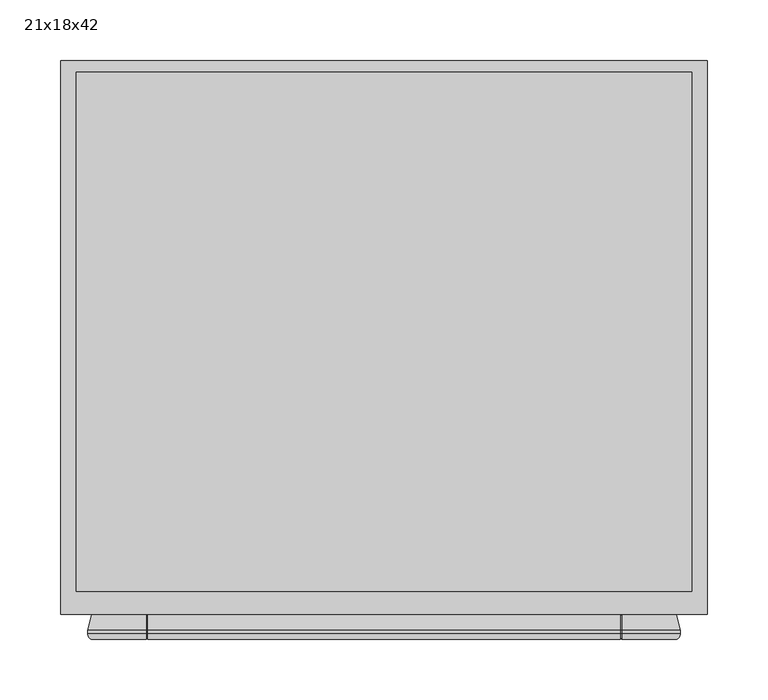
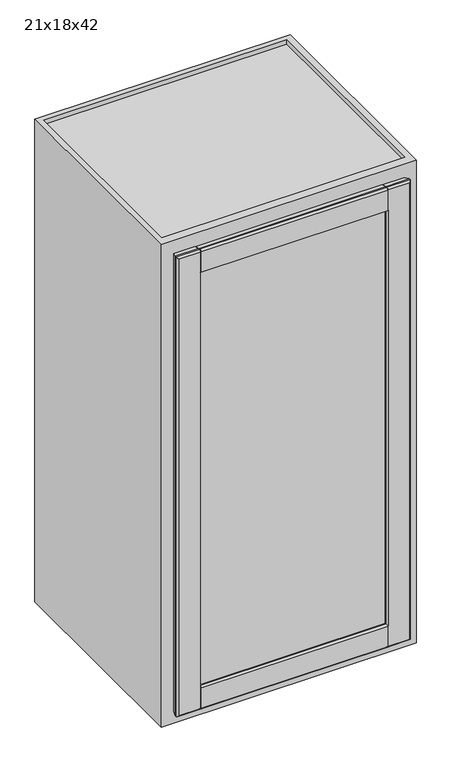
"""IFC4 building model written with IfcOpenShell, lengths in millimetres: furniture geometry, Cabinet-Wall-Merillat-Single_Door-Marlin : 21x18x42."""

import ifcopenshell
import ifcopenshell.guid

model = None  # the IFC model being written
_history = None  # IfcOwnerHistory: only IFC2X3 demands one
_inside = {}  # id of a spatial element -> (the spatial element, [elements in it])
_under = {}  # id of a project, library or spatial element -> (it, [spatial elements below it])
_declared = {}  # id of a project -> (the project, [libraries it declares])
_typed = {}  # id of a type object -> (the type object, [elements of that type])
_made_of = {}  # id of a material, layer set ... -> (it, [elements and type objects made of it])


def new_model(schema):
    """Start an empty IFC model of exactly this schema.

    Asked for "IFC4X3", IfcOpenShell would pick the latest addendum, in which some entities
    have other attributes; the version numbers below select the first issue.
    IFC2X3 requires an IfcOwnerHistory on every rooted entity: one is made here for all.
    """
    global model, _history
    if schema == "IFC4X3":
        model = ifcopenshell.file(schema_version=(4, 3, 0, 0))
    else:
        model = ifcopenshell.file(schema=schema)
    _inside.clear()
    _under.clear()
    _declared.clear()
    _typed.clear()
    _made_of.clear()
    _history = None
    if model.schema == "IFC2X3":
        org = make("IfcOrganization", Name="unknown")
        user = make(
            "IfcPersonAndOrganization",
            ThePerson=make("IfcPerson", FamilyName="unknown"),
            TheOrganization=org,
        )
        app = make(
            "IfcApplication",
            ApplicationDeveloper=org,
            Version="unknown",
            ApplicationFullName="unknown",
            ApplicationIdentifier="unknown",
        )
        _history = make(
            "IfcOwnerHistory",
            OwningUser=user,
            OwningApplication=app,
            ChangeAction="ADDED",
            CreationDate=0,
        )
    return model


def make(cls, **values):
    """One entity of the class cls with the attributes given. An attribute that is None is left unset."""
    return model.create_entity(
        cls, **{name: value for name, value in values.items() if value is not None}
    )


def rooted(cls, **values):
    """An entity with a GlobalId (a new one), such as an element, a storey or a relation."""
    return make(cls, GlobalId=ifcopenshell.guid.new(), OwnerHistory=_history, **values)


def si_unit(unit_type, name, prefix=None):
    """IfcSIUnit, for example si_unit("LENGTHUNIT", "METRE", prefix="MILLI")."""
    return make("IfcSIUnit", UnitType=unit_type, Prefix=prefix, Name=name)


def assignment(units):
    """IfcUnitAssignment: the units of a project."""
    return None if units is None else make("IfcUnitAssignment", Units=units)


def point(xyz):
    """IfcCartesianPoint."""
    return None if xyz is None else make("IfcCartesianPoint", Coordinates=xyz)


def direction(xyz):
    """IfcDirection."""
    return None if xyz is None else make("IfcDirection", DirectionRatios=xyz)


def frame(location, z_axis=None, x_axis=None):
    """IfcAxis2Placement3D, a coordinate frame: its origin and axes. An axis left out is left unset."""
    return make(
        "IfcAxis2Placement3D",
        Location=point(location),
        Axis=direction(z_axis),
        RefDirection=direction(x_axis),
    )


def origin():
    """The frame at (0, 0, 0) with its axes left unset."""
    return frame((0.0, 0.0, 0.0))


def place(relative_to, where):
    """IfcLocalPlacement: puts the frame where relative to a parent placement (None: the world)."""
    return make(
        "IfcLocalPlacement", PlacementRelTo=relative_to, RelativePlacement=where
    )


def context(
    kind, dimensions, precision=None, world=None, true_north=None, identifier=None
):
    """IfcGeometricRepresentationContext, for example the 3D "Model" context."""
    return make(
        "IfcGeometricRepresentationContext",
        ContextIdentifier=identifier,
        ContextType=kind,
        CoordinateSpaceDimension=dimensions,
        Precision=precision,
        WorldCoordinateSystem=world,
        TrueNorth=true_north,
    )


def project(units=None, contexts=None):
    """IfcProject with its units and contexts."""
    return rooted(
        "IfcProject",
        Name="project",
        RepresentationContexts=contexts,
        UnitsInContext=assignment(units),
    )


def spatial(cls, under=None, at=None, **own):
    """A site, building, storey or space (cls), placed at a placement, below another one or the project."""
    s = rooted(cls, ObjectPlacement=at, **own)
    if under is not None:
        _under.setdefault(under.id(), (under, []))[1].append(s)
    return s


def polyline(points):
    """IfcPolyline through the points."""
    return make("IfcPolyline", Points=[point(p) for p in points])


def circle_curve(where, radius):
    """IfcCircle in the frame where."""
    return make("IfcCircle", Position=where, Radius=radius)


def ellipse_curve(where, semi_axis1, semi_axis2):
    """IfcEllipse in the frame where."""
    return make(
        "IfcEllipse", Position=where, SemiAxis1=semi_axis1, SemiAxis2=semi_axis2
    )


def outline(outer, holes=None, kind="AREA"):
    """IfcArbitraryClosedProfileDef: a profile drawn as a closed curve; with holes, ...WithVoids."""
    if holes is None:
        return make("IfcArbitraryClosedProfileDef", ProfileType=kind, OuterCurve=outer)
    return make(
        "IfcArbitraryProfileDefWithVoids",
        ProfileType=kind,
        OuterCurve=outer,
        InnerCurves=holes,
    )


def extrude(swept, where, along, depth):
    """IfcExtrudedAreaSolid: the profile swept, set in the frame where, extruded along a direction by depth."""
    return make(
        "IfcExtrudedAreaSolid",
        SweptArea=swept,
        Position=where,
        ExtrudedDirection=direction(along),
        Depth=depth,
    )


def faces_of(points, faces, orient=None, outer=None):
    """IfcFace entities. A face is a list of loops; a loop is a list of indices into points, from 0.

    orient and outer hold one flag for each loop. By default every Orientation is true, the
    first loop of a face is its IfcFaceOuterBound and the others are IfcFaceBound.
    """
    made = []
    for i, loops in enumerate(faces):
        bounds = []
        for j, loop in enumerate(loops):
            is_outer = j == 0 if outer is None else outer[i][j]
            bounds.append(
                make(
                    "IfcFaceOuterBound" if is_outer else "IfcFaceBound",
                    Bound=make("IfcPolyLoop", Polygon=[points[k] for k in loop]),
                    Orientation=True if orient is None else orient[i][j],
                )
            )
        made.append(make("IfcFace", Bounds=bounds))
    return made


def faceted_brep(points, faces, orient=None, outer=None, voids=None):
    """IfcFacetedBrep: a solid bounded by flat faces; with voids (closed shells), ...WithVoids."""
    shared = [point(p) for p in points]
    hull = make("IfcClosedShell", CfsFaces=faces_of(shared, faces, orient, outer))
    if voids is None:
        return make("IfcFacetedBrep", Outer=hull)
    return make(
        "IfcFacetedBrepWithVoids",
        Outer=hull,
        Voids=[
            make(cls, CfsFaces=faces_of(shared, fs, o, b)) for cls, fs, o, b in voids
        ],
    )


def shape(context_of_items, identifier, shape_type, items):
    """IfcShapeRepresentation: the items that make up one representation, for example the "Body"."""
    return make(
        "IfcShapeRepresentation",
        ContextOfItems=context_of_items,
        RepresentationIdentifier=identifier,
        RepresentationType=shape_type,
        Items=items,
    )


def source(mapping_origin, context_of_items, identifier, shape_type, items):
    """IfcRepresentationMap: a shape defined once, which mapped items show again and again."""
    return make(
        "IfcRepresentationMap",
        MappingOrigin=mapping_origin,
        MappedRepresentation=shape(context_of_items, identifier, shape_type, items),
    )


def transform(
    local_origin,
    x_axis=None,
    y_axis=None,
    z_axis=None,
    scale=None,
    scale2=None,
    scale3=None,
    uniform=True,
):
    """IfcCartesianTransformationOperator3D, or its non-uniform kind. x_axis, y_axis, z_axis: its Axis1, 2, 3."""
    if uniform:
        return make(
            "IfcCartesianTransformationOperator3D",
            Axis1=direction(x_axis),
            Axis2=direction(y_axis),
            LocalOrigin=point(local_origin),
            Scale=scale,
            Axis3=direction(z_axis),
        )
    return make(
        "IfcCartesianTransformationOperator3DnonUniform",
        Axis1=direction(x_axis),
        Axis2=direction(y_axis),
        LocalOrigin=point(local_origin),
        Scale=scale,
        Axis3=direction(z_axis),
        Scale2=scale2,
        Scale3=scale3,
    )


def mapped(mapping_source, mapping_target):
    """IfcMappedItem: shows the shape of a source again, moved by a transform."""
    return make(
        "IfcMappedItem", MappingSource=mapping_source, MappingTarget=mapping_target
    )


def made_of(thing, what):
    """Note that an element or type object is made of a material, layer set ...; save() writes the relation."""
    if what is not None:
        _made_of.setdefault(what.id(), (what, []))[1].append(thing)
    return thing


def element(
    cls,
    number,
    at=None,
    inside=None,
    cuts=None,
    type_object=None,
    material=None,
    context=None,
    identifier="Body",
    shape_type=None,
    held_by="IfcProductDefinitionShape",
    body=None,
    shapes=None,
    **own,
):
    """One element of the class cls, such as IfcWall. Its Tag is "e" and its number.

    at: its placement. inside: the storey or other place that contains it. cuts: it is an
    opening in that element (IfcRelVoidsElement). A single representation is given by context,
    identifier, shape_type and body (its items); several are given by shapes. held_by: the class
    of the entity that holds the representations. save() writes the other relations.
    """
    e = rooted(cls, Tag="e%d" % number, ObjectPlacement=at, **own)
    if body is not None:
        shapes = [shape(context, identifier, shape_type, body)]
    if shapes is not None:
        e.Representation = make(held_by, Representations=shapes)
    if inside is not None:
        _inside.setdefault(inside.id(), (inside, []))[1].append(e)
    if cuts is not None:
        rooted(
            "IfcRelVoidsElement", RelatingBuildingElement=cuts, RelatedOpeningElement=e
        )
    if type_object is not None:
        _typed.setdefault(type_object.id(), (type_object, []))[1].append(e)
    return made_of(e, material)


def aggregate(whole, parts):
    """IfcRelAggregates: a whole, such as a stair, and the parts it consists of."""
    return rooted("IfcRelAggregates", RelatingObject=whole, RelatedObjects=parts)


def save(model, path):
    """Write the relations noted so far, then the file.

    IfcRelAggregates (storeys below a building ...), IfcRelContainedInSpatialStructure (elements
    in a storey), IfcRelDefinesByType, IfcRelAssociatesMaterial and IfcRelDeclares: one each for
    every whole, place, type object, material and project.
    """
    for whole, parts in _under.values():
        aggregate(whole, parts)
    for where, things in _inside.values():
        rooted(
            "IfcRelContainedInSpatialStructure",
            RelatedElements=things,
            RelatingStructure=where,
        )
    for kind, things in _typed.values():
        rooted("IfcRelDefinesByType", RelatedObjects=things, RelatingType=kind)
    for what, things in _made_of.values():
        rooted("IfcRelAssociatesMaterial", RelatedObjects=things, RelatingMaterial=what)
    for by, libraries in _declared.values():
        rooted("IfcRelDeclares", RelatingContext=by, RelatedDefinitions=libraries)
    model.write(path)


def plane_surface(at):
    """IfcPlane: the flat surface through the origin of the frame at, square to its z axis."""
    return make("IfcPlane", Position=at)


def cylinder_surface(at, radius):
    """IfcCylindricalSurface: all points at the distance radius from the z axis of the frame at."""
    return make("IfcCylindricalSurface", Position=at, Radius=radius)


def advanced_brep(points, edges, surfaces, faces):
    """IfcAdvancedBrep: a solid bounded by faces that lie on surfaces and meet in shared edges.

    An edge is (start, end): straight between two places in points (the first is 0);
    or (start, end, curve); or (start, end, curve, False) where it runs against its curve.
    A face is (place in surfaces, loops), or (place, loops, False) where it looks against
    its surface's normal. A loop lists edges by number (the first is 1), with a minus sign
    where the edge is run from its end to its start. The first loop is the outer one.
    """
    corners = [point(p) for p in points]
    vertices = [make("IfcVertexPoint", VertexGeometry=c) for c in corners]
    made = []
    for start, end, *more in edges:
        made.append(
            make(
                "IfcEdgeCurve",
                EdgeStart=vertices[start],
                EdgeEnd=vertices[end],
                EdgeGeometry=more[0] if more else make("IfcPolyline", Points=[corners[start], corners[end]]),
                SameSense=more[1] if len(more) > 1 else True,
            )
        )
    hull = []
    for where, loops, *sense in faces:
        bounds = []
        for j, loop in enumerate(loops):
            ring = [make("IfcOrientedEdge", EdgeElement=made[abs(k) - 1], Orientation=k > 0) for k in loop]
            bounds.append(
                make(
                    "IfcFaceOuterBound" if j == 0 else "IfcFaceBound",
                    Bound=make("IfcEdgeLoop", EdgeList=ring),
                    Orientation=True,
                )
            )
        hull.append(make("IfcAdvancedFace", Bounds=bounds, FaceSurface=surfaces[where], SameSense=sense[0] if sense else True))
    return make("IfcAdvancedBrep", Outer=make("IfcClosedShell", CfsFaces=hull))


def furniture_21x18x42_ea13cc69(model_context):
    return source(origin(), model_context, "Body", "SolidModel", [
        advanced_brep(
        [(-214.7038372, -534.9621, 2108.2), (-214.7038372, -534.9621, 1092.2), (-211.6073447, -539.4325, 1095.2964925), (-211.6073447, -539.4325, 2105.1035075), (-214.7038372, -532.1935, 2108.2), (-214.7038372, -532.1935, 1092.2), (-211.1986372, -519.1125, 2104.6948), (-211.1986372, -519.1125, 1095.7052), (-166.5026744, -519.1125, 2059.9988372), (-166.1325427, -519.90625, 2059.6287055), (-164.0513837, -524.36931, 2057.5475465), (-164.0513837, -524.36931, 1142.8524535), (-166.1325427, -519.90625, 1140.7712945), (-166.5026744, -519.1125, 1140.4011628), (-165.4511532, -526.6094093, 2058.947316), (-165.4511532, -526.6094093, 1141.452684), (-179.7788372, -526.8595, 2073.275), (-179.7788372, -526.8595, 1127.125), (-179.7788372, -531.6855, 2073.275), (-179.7788372, -531.6855, 1127.125), (-165.4511532, -531.9355907, 2058.947316), (-165.4511532, -531.9355907, 1141.452684), (-164.0513837, -534.17569, 2057.5475465), (-164.0513837, -534.17569, 1142.8524535), (-166.1325427, -538.63875, 2059.6287055), (-166.499807, -539.4263508, 2059.9959698), (-166.5026744, -539.4325, 1140.4011628), (-166.1325427, -538.63875, 1140.7712945), (271.1496703, -539.4325, 1095.2964925), (226.0819441, -539.4325, 1095.2964925), (226.0819441, -534.9621, 1092.2), (274.2461628, -534.9621, 1092.2), (-166.499807, -534.9621, 1092.2), (-166.499807, -539.4325, 1095.2964925), (-164.912307, -534.9621, 1092.2), (224.4944441, -534.9621, 1092.2), (224.4944441, -539.4325, 1095.2964925), (-164.912307, -539.4325, 1095.2964925), (226.0819441, -532.1935, 1092.2), (274.2461628, -532.1935, 1092.2), (-166.499807, -532.1935, 1092.2), (-164.912307, -532.1935, 1092.2), (224.4944441, -532.1935, 1092.2), (226.0819441, -519.1125, 1095.7052), (270.7409628, -519.1125, 1095.7052), (-166.499807, -519.1125, 1095.7052), (-164.912307, -519.1125, 1095.7052), (224.4944441, -519.1125, 1095.7052), (223.5937093, -524.36931, 1142.8524535), (225.6748683, -519.90625, 1140.7712945), (224.4944441, -519.90625, 1140.7712945), (224.4944441, -519.1125, 1140.4011628), (-164.912307, -519.1125, 1140.4011628), (-164.912307, -519.90625, 1140.7712945), (224.9934787, -526.6094093, 1141.452684), (239.3211628, -526.8595, 1127.125), (239.3211628, -531.6855, 1127.125), (224.9934787, -531.9355907, 1141.452684), (223.5937093, -534.17569, 1142.8524535), (-164.912307, -538.63875, 1140.7712945), (-164.912307, -539.4325, 1140.4011628), (224.4944441, -539.4325, 1140.4011628), (224.4944441, -538.63875, 1140.7712945), (225.6748683, -538.63875, 1140.7712945), (274.2461628, -534.9621, 2108.2), (271.1496703, -539.4325, 2105.1035075), (274.2461628, -532.1935, 2108.2), (270.7409628, -519.1125, 2104.6948), (226.045, -519.1125, 1140.4011628), (223.5937093, -524.36931, 2057.5475465), (225.6748683, -519.90625, 2059.6287055), (226.045, -519.1125, 2059.9988372), (224.9934787, -526.6094093, 2058.947316), (239.3211628, -526.8595, 2073.275), (239.3211628, -531.6855, 2073.275), (224.9934787, -531.9355907, 2058.947316), (223.5937093, -534.17569, 2057.5475465), (226.045, -539.4325, 1140.4011628), (226.045, -539.4325, 2059.9988372), (225.6748683, -538.63875, 2059.6287055), (-166.499807, -539.4325, 2105.1035075), (-166.499807, -534.9621, 2108.2), (226.0819441, -534.9621, 2108.2), (226.0819441, -539.4325, 2105.1035075), (224.4944441, -534.9621, 2108.2), (-164.912307, -534.9621, 2108.2), (-164.912307, -539.4325, 2105.1035075), (224.4944441, -539.4325, 2105.1035075), (-166.499807, -532.1935, 2108.2), (226.0819441, -532.1935, 2108.2), (224.4944441, -532.1935, 2108.2), (-164.912307, -532.1935, 2108.2), (-166.499807, -519.1125, 2104.6948), (226.0819441, -519.1125, 2104.6948), (224.4944441, -519.1125, 2104.6948), (-164.912307, -519.1125, 2104.6948), (224.4944441, -519.1125, 2059.9988372), (-164.912307, -519.1125, 2059.9988372), (-164.912307, -519.90625, 2059.6287055), (224.4944441, -519.90625, 2059.6287055), (224.4944441, -538.63875, 2059.6287055), (224.4944441, -539.4325, 2059.9988372), (-164.912307, -539.4325, 2059.9988372), (-164.912307, -538.63875, 2059.6287055), (224.4944441, -538.63875, 2104.9526052), (224.4944441, -534.9621, 2107.40625), (224.4944441, -532.2980037, 2107.40625), (224.4944441, -519.90625, 2104.0857412), (226.0819441, -519.90625, 2059.6287055), (226.0819441, -519.90625, 2104.0857412), (226.0819441, -532.2980037, 2107.40625), (226.0819441, -534.9621, 2107.40625), (226.0819441, -538.63875, 2104.9526052), (226.0819441, -538.63875, 2059.6287055), (-166.499807, -538.63875, 2059.6287055), (-166.499807, -538.63875, 2104.9526052), (-166.499807, -534.9621, 2107.40625), (-166.499807, -532.2980037, 2107.40625), (-166.499807, -519.90625, 2104.0857412), (-166.499807, -519.90625, 2059.6287055), (-164.912307, -519.90625, 2104.0857412), (-164.912307, -532.2980037, 2107.40625), (-164.912307, -534.9621, 2107.40625), (-164.912307, -538.63875, 2104.9526052), (-166.499807, -519.90625, 1140.7712945), (-166.499807, -519.90625, 1096.3142588), (-166.499807, -532.2980037, 1092.99375), (-166.499807, -534.9621, 1092.99375), (-166.499807, -538.63875, 1095.4473948), (-166.499807, -538.63875, 1140.7712945), (-164.912307, -538.63875, 1095.4473948), (-164.912307, -534.9621, 1092.99375), (-164.912307, -532.2980037, 1092.99375), (-164.912307, -519.90625, 1096.3142588), (224.4944441, -519.90625, 1096.3142588), (224.4944441, -532.2980037, 1092.99375), (224.4944441, -534.9621, 1092.99375), (224.4944441, -538.63875, 1095.4473948), (226.0819441, -538.63875, 1140.7712945), (226.0819441, -538.63875, 1095.4473948), (226.0819441, -534.9621, 1092.99375), (226.0819441, -532.2980037, 1092.99375), (226.0819441, -519.90625, 1096.3142588), (226.0819441, -519.90625, 1140.7712945)],
        [
            (0, 1),
            (1, 2, ellipse_curve(frame((-209.9286372, -534.9621, 1096.9752), z_axis=(-0.7071067811865475, 0.0, 0.7071067811865475), x_axis=(0.7071067811865474, 0.0, 0.7071067811865476)), 6.7531526, 4.7752)),
            (2, 3),
            (3, 0, ellipse_curve(frame((-209.9286372, -534.9621, 2103.4248), z_axis=(-0.7071067811865475, 0.0, -0.7071067811865475), x_axis=(-0.7071067811865474, 0.0, 0.7071067811865476)), 6.7531526, 4.7752)),
            (0, 4),
            (4, 5),
            (5, 1),
            (4, 6),
            (6, 7),
            (7, 5),
            (8, 9),
            (9, 10),
            (10, 11),
            (11, 12),
            (12, 13),
            (13, 8),
            (10, 14, ellipse_curve(frame((-165.4786372, -525.0348492, 2058.9748), z_axis=(-0.7071067811865475, 0.0, -0.7071067811865475), x_axis=(-0.7071067811865474, 0.0, 0.7071067811865476)), 2.2271035, 1.5748)),
            (14, 15),
            (15, 11, ellipse_curve(frame((-165.4786372, -525.0348492, 1141.4252), z_axis=(-0.7071067811865475, 0.0, 0.7071067811865475), x_axis=(0.7071067811865474, 0.0, 0.7071067811865476)), 2.2271035, 1.5748)),
            (14, 16),
            (16, 17),
            (17, 15),
            (16, 18),
            (18, 19),
            (19, 17),
            (18, 20),
            (20, 21),
            (21, 19),
            (20, 22, ellipse_curve(frame((-165.4786372, -533.5101508, 2058.9748), z_axis=(-0.7071067811865475, 0.0, -0.7071067811865475), x_axis=(-0.7071067811865474, 0.0, 0.7071067811865476)), 2.2271035, 1.5748)),
            (22, 23),
            (23, 21, ellipse_curve(frame((-165.4786372, -533.5101508, 1141.4252), z_axis=(-0.7071067811865475, 0.0, 0.7071067811865475), x_axis=(0.7071067811865474, 0.0, 0.7071067811865476)), 2.2271035, 1.5748)),
            (22, 24),
            (24, 25),
            (25, 26),
            (26, 27),
            (27, 23),
            (28, 29),
            (29, 30, circle_curve(frame((226.0819441, -534.9621, 1096.9752), z_axis=(1.0, 0.0, 0.0), x_axis=(0.0, 1.0, 0.0)), 4.7752)),
            (30, 31),
            (31, 28, ellipse_curve(frame((269.4709628, -534.9621, 1096.9752), z_axis=(-0.7071067811865475, 0.0, -0.7071067811865475), x_axis=(-0.7071067811865476, 0.0, 0.7071067811865474)), 6.7531526, 4.7752)),
            (1, 32),
            (32, 33, circle_curve(frame((-166.499807, -534.9621, 1096.9752), z_axis=(-1.0, 0.0, 0.0), x_axis=(0.0, 1.0, 0.0)), 4.7752)),
            (33, 2),
            (34, 35),
            (35, 36, circle_curve(frame((224.4944441, -534.9621, 1096.9752), z_axis=(-1.0, 0.0, 0.0), x_axis=(0.0, 1.0, 0.0)), 4.7752)),
            (36, 37),
            (37, 34, circle_curve(frame((-164.912307, -534.9621, 1096.9752), z_axis=(1.0, 0.0, 0.0), x_axis=(0.0, 1.0, 0.0)), 4.7752)),
            (30, 38),
            (38, 39),
            (39, 31),
            (5, 40),
            (40, 32),
            (41, 42),
            (42, 35),
            (34, 41),
            (38, 43),
            (43, 44),
            (44, 39),
            (7, 45),
            (45, 40),
            (46, 47),
            (47, 42),
            (41, 46),
            (48, 49),
            (49, 50),
            (50, 51),
            (51, 52),
            (52, 53),
            (53, 12),
            (11, 48),
            (15, 54),
            (54, 48, ellipse_curve(frame((225.0209628, -525.0348492, 1141.4252), z_axis=(-0.7071067811865475, 0.0, -0.7071067811865475), x_axis=(-0.7071067811865476, 0.0, 0.7071067811865474)), 2.2271035, 1.5748)),
            (17, 55),
            (55, 54),
            (19, 56),
            (56, 55),
            (21, 57),
            (57, 56),
            (23, 58),
            (58, 57, ellipse_curve(frame((225.0209628, -533.5101508, 1141.4252), z_axis=(-0.7071067811865475, 0.0, -0.7071067811865475), x_axis=(-0.7071067811865476, 0.0, 0.7071067811865474)), 2.2271035, 1.5748)),
            (27, 59),
            (59, 60),
            (60, 61),
            (61, 62),
            (62, 63),
            (63, 58),
            (31, 64),
            (64, 65, ellipse_curve(frame((269.4709628, -534.9621, 2103.4248), z_axis=(0.7071067811865475, 0.0, -0.7071067811865475), x_axis=(-0.7071067811865474, 0.0, -0.7071067811865476)), 6.7531526, 4.7752)),
            (65, 28),
            (39, 66),
            (66, 64),
            (44, 67),
            (67, 66),
            (68, 49),
            (48, 69),
            (69, 70),
            (70, 71),
            (71, 68),
            (54, 72),
            (72, 69, ellipse_curve(frame((225.0209628, -525.0348492, 2058.9748), z_axis=(0.7071067811865475, 0.0, -0.7071067811865475), x_axis=(-0.7071067811865474, 0.0, -0.7071067811865476)), 2.2271035, 1.5748)),
            (55, 73),
            (73, 72),
            (56, 74),
            (74, 73),
            (57, 75),
            (75, 74),
            (58, 76),
            (76, 75, ellipse_curve(frame((225.0209628, -533.5101508, 2058.9748), z_axis=(0.7071067811865475, 0.0, -0.7071067811865475), x_axis=(-0.7071067811865474, 0.0, -0.7071067811865476)), 2.2271035, 1.5748)),
            (63, 77),
            (77, 78),
            (78, 79),
            (79, 76),
            (3, 80),
            (80, 81, circle_curve(frame((-166.499807, -534.9621, 2103.4248), z_axis=(-1.0, 0.0, 0.0), x_axis=(0.0, 1.0, 0.0)), 4.7752)),
            (81, 0),
            (64, 82),
            (82, 83, circle_curve(frame((226.0819441, -534.9621, 2103.4248), z_axis=(1.0, 0.0, 0.0), x_axis=(0.0, 1.0, 0.0)), 4.7752)),
            (83, 65),
            (84, 85),
            (85, 86, circle_curve(frame((-164.912307, -534.9621, 2103.4248), z_axis=(1.0, 0.0, 0.0), x_axis=(0.0, 1.0, 0.0)), 4.7752)),
            (86, 87),
            (87, 84, circle_curve(frame((224.4944441, -534.9621, 2103.4248), z_axis=(-1.0, 0.0, 0.0), x_axis=(0.0, 1.0, 0.0)), 4.7752)),
            (81, 88),
            (88, 4),
            (66, 89),
            (89, 82),
            (90, 91),
            (91, 85),
            (84, 90),
            (88, 92),
            (92, 6),
            (67, 93),
            (93, 89),
            (94, 95),
            (95, 91),
            (90, 94),
            (51, 47),
            (46, 52),
            (92, 8),
            (13, 45),
            (43, 68),
            (71, 93),
            (96, 97),
            (97, 95),
            (94, 96),
            (9, 98),
            (98, 97),
            (96, 99),
            (99, 70),
            (69, 10),
            (72, 14),
            (73, 16),
            (74, 18),
            (75, 20),
            (76, 22),
            (79, 100),
            (100, 101),
            (101, 102),
            (102, 103),
            (103, 24),
            (33, 26),
            (25, 80),
            (36, 61),
            (60, 37),
            (83, 78),
            (77, 29),
            (86, 102),
            (101, 87),
            (100, 104),
            (104, 105, circle_curve(frame((224.4944441, -534.9621, 2103.4248), z_axis=(-1.0, 0.0, 0.0), x_axis=(0.0, 0.0, 1.0)), 3.98145)),
            (105, 106),
            (106, 107),
            (107, 99),
            (71, 108),
            (108, 109),
            (109, 110),
            (110, 111),
            (111, 112, circle_curve(frame((226.0819441, -534.9621, 2103.4248), z_axis=(1.0, 0.0, 0.0), x_axis=(0.0, 0.0, 1.0)), 3.98145)),
            (112, 113),
            (113, 78),
            (113, 79),
            (112, 104),
            (111, 105),
            (110, 106),
            (109, 107),
            (108, 70),
            (25, 114),
            (114, 115),
            (115, 116, circle_curve(frame((-166.499807, -534.9621, 2103.4248), z_axis=(-1.0, 0.0, 0.0), x_axis=(0.0, 0.0, 1.0)), 3.98145)),
            (116, 117),
            (117, 118),
            (118, 119),
            (119, 8),
            (98, 120),
            (120, 121),
            (121, 122),
            (122, 123, circle_curve(frame((-164.912307, -534.9621, 2103.4248), z_axis=(1.0, 0.0, 0.0), x_axis=(0.0, 0.0, 1.0)), 3.98145)),
            (123, 103),
            (24, 114),
            (123, 115),
            (122, 116),
            (121, 117),
            (120, 118),
            (9, 119),
            (13, 124),
            (124, 125),
            (125, 126),
            (126, 127),
            (127, 128, circle_curve(frame((-166.499807, -534.9621, 1096.9752), z_axis=(-1.0, 0.0, 0.0), x_axis=(0.0, 0.0, 1.0)), 3.98145)),
            (128, 129),
            (129, 26),
            (59, 130),
            (130, 131, circle_curve(frame((-164.912307, -534.9621, 1096.9752), z_axis=(1.0, 0.0, 0.0), x_axis=(0.0, 0.0, 1.0)), 3.98145)),
            (131, 132),
            (132, 133),
            (133, 53),
            (12, 124),
            (133, 125),
            (132, 126),
            (131, 127),
            (130, 128),
            (27, 129),
            (50, 134),
            (134, 135),
            (135, 136),
            (136, 137, circle_curve(frame((224.4944441, -534.9621, 1096.9752), z_axis=(-1.0, 0.0, 0.0), x_axis=(0.0, 0.0, 1.0)), 3.98145)),
            (137, 62),
            (138, 139),
            (139, 140, circle_curve(frame((226.0819441, -534.9621, 1096.9752), z_axis=(1.0, 0.0, 0.0), x_axis=(0.0, 0.0, 1.0)), 3.98145)),
            (140, 141),
            (141, 142),
            (142, 143),
            (143, 68),
            (77, 138),
            (63, 138),
            (143, 49),
            (142, 134),
            (141, 135),
            (140, 136),
            (139, 137),
        ],
        [
            cylinder_surface(frame((-209.9286372, -534.9621, 2108.2), z_axis=(0.0, 0.0, 1.0), x_axis=(0.0, 1.0, 0.0)), 4.7752),
            plane_surface(frame((-214.7038372, -534.9621, 2108.2), z_axis=(-1.0, 0.0, 0.0), x_axis=(0.0, 0.0, -1.0))),
            plane_surface(frame((-214.7038372, -532.1935, 2108.2), z_axis=(-0.9659229350723619, 0.25882983502910506, 0.0), x_axis=(0.0, 0.0, -1.0))),
            plane_surface(frame((-166.5026744, -519.1125, 2059.9988372), z_axis=(0.9063077870366099, 0.4226182617407856, 0.0), x_axis=(0.0, 0.0, -1.0))),
            cylinder_surface(frame((-165.4786372, -525.0348492, 2108.2), z_axis=(0.0, 0.0, 1.0000000000000002), x_axis=(0.01745240643729364, -0.9998476951563912, 0.0)), 1.5748),
            plane_surface(frame((-165.4511532, -526.6094093, 2058.947316), z_axis=(0.017452406437322144, -0.9998476951563906, 0.0), x_axis=(0.0, 0.0, -1.0))),
            plane_surface(frame((-179.7788372, -526.8595, 2073.275), z_axis=(1.0, 0.0, 0.0), x_axis=(0.0, 0.0, -1.0))),
            plane_surface(frame((-179.7788372, -531.6855, 2073.275), z_axis=(0.01745240643727848, 0.9998476951563914, 0.0), x_axis=(0.0, 0.0, -1.0))),
            cylinder_surface(frame((-165.4786372, -533.5101508, 2108.2), z_axis=(0.0, 0.0, 1.0000000000000002), x_axis=(0.9063077870367326, -0.42261826174052236, 0.0)), 1.5748),
            plane_surface(frame((-164.0513837, -534.17569, 2057.5475465), z_axis=(0.9063077870366333, -0.4226182617407352, 0.0), x_axis=(0.0, 0.0, -1.0))),
            cylinder_surface(frame((-214.7038372, -534.9621, 1096.9752), z_axis=(-1.0, 0.0, 0.0), x_axis=(0.0, 1.0, 0.0)), 4.7752),
            plane_surface(frame((-214.7038372, -534.9621, 1092.2), z_axis=(0.0, 0.0, -1.0), x_axis=(1.0, 0.0, 0.0))),
            plane_surface(frame((-214.7038372, -532.1935, 1092.2), z_axis=(0.0, 0.2588298350291095, -0.9659229350723607), x_axis=(1.0, 0.0, 0.0))),
            plane_surface(frame((-166.5026744, -519.1125, 1140.4011628), z_axis=(0.0, 0.42261826174078143, 0.9063077870366119), x_axis=(1.0, 0.0, 0.0))),
            cylinder_surface(frame((-214.7038372, -525.0348492, 1141.4252), z_axis=(-1.0000000000000002, 0.0, 0.0), x_axis=(0.0, -0.9998476951563913, 0.017452406437289025)), 1.5748),
            plane_surface(frame((-165.4511532, -526.6094093, 1141.452684), z_axis=(0.0, -0.9998476951563907, 0.01745240643731753), x_axis=(1.0, 0.0, 0.0))),
            plane_surface(frame((-179.7788372, -526.8595, 1127.125), z_axis=(0.0, 0.0, 1.0), x_axis=(1.0, 0.0, 0.0))),
            plane_surface(frame((-179.7788372, -531.6855, 1127.125), z_axis=(0.0, 0.9998476951563913, 0.017452406437283095), x_axis=(1.0, 0.0, 0.0))),
            cylinder_surface(frame((-214.7038372, -533.5101508, 1141.4252), z_axis=(-1.0000000000000002, 0.0, 0.0), x_axis=(0.0, -0.4226182617405265, 0.9063077870367306)), 1.5748),
            plane_surface(frame((-164.0513837, -534.17569, 1142.8524535), z_axis=(0.0, -0.4226182617407394, 0.9063077870366314), x_axis=(1.0, 0.0, 0.0))),
            cylinder_surface(frame((269.4709628, -534.9621, 1092.2), z_axis=(0.0, 0.0, -1.0), x_axis=(0.0, 1.0, 0.0)), 4.7752),
            plane_surface(frame((274.2461628, -534.9621, 1092.2), z_axis=(1.0, 0.0, 0.0), x_axis=(0.0, 0.0, 1.0))),
            plane_surface(frame((274.2461628, -532.1935, 1092.2), z_axis=(0.9659229350723619, 0.25882983502910506, 0.0), x_axis=(0.0, 0.0, 1.0))),
            plane_surface(frame((226.045, -519.1125, 1140.4011628), z_axis=(-0.9063077870366099, 0.4226182617407856, 0.0), x_axis=(0.0, 0.0, 1.0))),
            cylinder_surface(frame((225.0209628, -525.0348492, 1092.2), z_axis=(0.0, 0.0, -1.0000000000000002), x_axis=(-0.01745240643729364, -0.9998476951563912, 0.0)), 1.5748),
            plane_surface(frame((224.9934787, -526.6094093, 1141.452684), z_axis=(-0.017452406437322144, -0.9998476951563906, 0.0), x_axis=(0.0, 0.0, 1.0))),
            plane_surface(frame((239.3211628, -526.8595, 1127.125), z_axis=(-1.0, 0.0, 0.0), x_axis=(0.0, 0.0, 1.0))),
            plane_surface(frame((239.3211628, -531.6855, 1127.125), z_axis=(-0.01745240643727848, 0.9998476951563914, 0.0), x_axis=(0.0, 0.0, 1.0))),
            cylinder_surface(frame((225.0209628, -533.5101508, 1092.2), z_axis=(0.0, 0.0, -1.0000000000000002), x_axis=(-0.9063077870367326, -0.42261826174052236, 0.0)), 1.5748),
            plane_surface(frame((223.5937093, -534.17569, 1142.8524535), z_axis=(-0.9063077870366333, -0.4226182617407352, 0.0), x_axis=(0.0, 0.0, 1.0))),
            cylinder_surface(frame((274.2461628, -534.9621, 2103.4248), z_axis=(1.0, 0.0, 0.0), x_axis=(0.0, 1.0, 0.0)), 4.7752),
            plane_surface(frame((274.2461628, -534.9621, 2108.2), z_axis=(0.0, 0.0, 1.0), x_axis=(-1.0, 0.0, 0.0))),
            plane_surface(frame((274.2461628, -532.1935, 2108.2), z_axis=(0.0, 0.2588298350291006, 0.9659229350723632), x_axis=(-1.0, 0.0, 0.0))),
            plane_surface(frame((270.7409628, -519.1125, 2104.6948), z_axis=(0.0, 1.0, 0.0), x_axis=(-1.0, 0.0, 0.0))),
            plane_surface(frame((226.045, -519.1125, 2059.9988372), z_axis=(0.0, 0.42261826174078976, -0.9063077870366079), x_axis=(-1.0, 0.0, 0.0))),
            cylinder_surface(frame((274.2461628, -525.0348492, 2058.9748), z_axis=(1.0000000000000002, 0.0, 0.0), x_axis=(0.0, -0.999847695156391, -0.017452406437298253)), 1.5748),
            plane_surface(frame((224.9934787, -526.6094093, 2058.947316), z_axis=(0.0, -0.9998476951563905, -0.01745240643732676), x_axis=(-1.0, 0.0, 0.0))),
            plane_surface(frame((239.3211628, -526.8595, 2073.275), z_axis=(0.0, 0.0, -1.0), x_axis=(-1.0, 0.0, 0.0))),
            plane_surface(frame((239.3211628, -531.6855, 2073.275), z_axis=(0.0, 0.9998476951563915, -0.017452406437273867), x_axis=(-1.0, 0.0, 0.0))),
            cylinder_surface(frame((274.2461628, -533.5101508, 2058.9748), z_axis=(1.0000000000000002, 0.0, 0.0), x_axis=(0.0, -0.4226182617405182, -0.9063077870367346)), 1.5748),
            plane_surface(frame((223.5937093, -534.17569, 2057.5475465), z_axis=(0.0, -0.422618261740731, -0.9063077870366353), x_axis=(-1.0, 0.0, 0.0))),
            plane_surface(frame((226.045, -539.4325, 2059.9988372), z_axis=(0.0, -1.0, 0.0), x_axis=(-1.0, 0.0, 0.0))),
            plane_surface(frame((224.4944441, -539.4325, 2059.9988372), z_axis=(1.0, 0.0, 0.0), x_axis=(0.0, 0.9063077870366119, -0.4226182617407812))),
            plane_surface(frame((226.0819441, -539.4325, 2059.9988372), z_axis=(-1.0, 0.0, 0.0), x_axis=(0.0, -0.9063077870366119, 0.4226182617407812))),
            plane_surface(frame((224.4944441, -539.4325, 2059.9988372), z_axis=(0.0, 0.4226182617407812, 0.9063077870366119), x_axis=(1.0, 0.0, 0.0))),
            plane_surface(frame((224.4944441, -538.63875, 2059.6287055), z_axis=(0.0, -1.0, 0.0), x_axis=(1.0, 0.0, 0.0))),
            cylinder_surface(frame((226.0819441, -534.9621, 2103.4248), z_axis=(1.0, 0.0, 0.0), x_axis=(0.0, 0.0, 1.0)), 3.98145),
            plane_surface(frame((224.4944441, -534.9621, 2107.40625), z_axis=(0.0, 0.0, 1.0), x_axis=(1.0, 0.0, 0.0))),
            plane_surface(frame((224.4944441, -532.2980037, 2107.40625), z_axis=(0.0, 0.25882983502916007, 0.9659229350723473), x_axis=(1.0, 0.0, 0.0))),
            plane_surface(frame((224.4944441, -519.90625, 2104.0857412), z_axis=(0.0, 1.0, 0.0), x_axis=(1.0, 0.0, 0.0))),
            plane_surface(frame((224.4944441, -519.90625, 2059.6287055), z_axis=(0.0, -0.4226182617408151, 0.906307787036596), x_axis=(1.0, 0.0, 0.0))),
            plane_surface(frame((-166.499807, -539.4325, 2059.9988372), z_axis=(1.0, 0.0, 0.0), x_axis=(0.0, 0.9063077870366119, -0.4226182617407812))),
            plane_surface(frame((-164.912307, -539.4325, 2059.9988372), z_axis=(-1.0, 0.0, 0.0), x_axis=(0.0, -0.9063077870366119, 0.4226182617407812))),
            plane_surface(frame((-166.499807, -539.4325, 2059.9988372), z_axis=(0.0, 0.4226182617407812, 0.9063077870366119), x_axis=(1.0, 0.0, 0.0))),
            plane_surface(frame((-166.499807, -538.63875, 2059.6287055), z_axis=(0.0, -1.0, 0.0), x_axis=(1.0, 0.0, 0.0))),
            cylinder_surface(frame((-164.912307, -534.9621, 2103.4248), z_axis=(1.0, 0.0, 0.0), x_axis=(0.0, 0.0, 1.0)), 3.98145),
            plane_surface(frame((-166.499807, -534.9621, 2107.40625), z_axis=(0.0, 0.0, 1.0), x_axis=(1.0, 0.0, 0.0))),
            plane_surface(frame((-166.499807, -532.2980037, 2107.40625), z_axis=(0.0, 0.25882983502916257, 0.9659229350723466), x_axis=(1.0, 0.0, 0.0))),
            plane_surface(frame((-166.499807, -519.90625, 2104.0857412), z_axis=(0.0, 1.0, 0.0), x_axis=(1.0, 0.0, 0.0))),
            plane_surface(frame((-166.499807, -519.90625, 2059.6287055), z_axis=(0.0, -0.42261826174081607, 0.9063077870365956), x_axis=(1.0, 0.0, 0.0))),
            plane_surface(frame((-166.499807, -534.9621, 1101.7504), z_axis=(1.0, 0.0, 0.0), x_axis=(0.0, -1.0, 0.0))),
            plane_surface(frame((-164.912307, -534.9621, 1101.7504), z_axis=(-1.0, 0.0, 0.0), x_axis=(0.0, 1.0, 0.0))),
            plane_surface(frame((-166.499807, -519.1125, 1140.4011628), z_axis=(0.0, -0.4226182617407898, -0.906307787036608), x_axis=(1.0, 0.0, 0.0))),
            plane_surface(frame((-166.499807, -519.90625, 1140.7712945), z_axis=(0.0, 1.0, 0.0), x_axis=(1.0, 0.0, 0.0))),
            plane_surface(frame((-166.499807, -519.90625, 1096.3142588), z_axis=(0.0, 0.2588298350294553, -0.9659229350722681), x_axis=(1.0, 0.0, 0.0))),
            plane_surface(frame((-166.499807, -532.2980037, 1092.99375), z_axis=(0.0, 0.0, -1.0), x_axis=(1.0, 0.0, 0.0))),
            cylinder_surface(frame((-164.912307, -534.9621, 1096.9752), z_axis=(1.0, 0.0, 0.0), x_axis=(0.0, 0.0, 1.0)), 3.98145),
            plane_surface(frame((-166.499807, -538.63875, 1095.4473948), z_axis=(0.0, -1.0, 0.0), x_axis=(1.0, 0.0, 0.0))),
            plane_surface(frame((-166.499807, -538.63875, 1140.7712945), z_axis=(0.0, 0.42261826174079614, -0.9063077870366049), x_axis=(1.0, 0.0, 0.0))),
            plane_surface(frame((224.4944441, -538.63875, 1140.7712945), z_axis=(1.0000000000000002, 0.0, 0.0), x_axis=(0.0, -0.9063077870366271, -0.4226182617407486))),
            plane_surface(frame((226.0819441, -538.63875, 1140.7712945), z_axis=(-1.0000000000000002, 0.0, 0.0), x_axis=(0.0, 0.9063077870366271, 0.4226182617407486))),
            plane_surface(frame((224.4944441, -538.63875, 1140.7712945), z_axis=(0.0, 0.4226182617407486, -0.9063077870366271), x_axis=(1.0, 0.0, 0.0))),
            plane_surface(frame((224.4944441, -519.1125, 1140.4011628), z_axis=(0.0, -0.4226182617407898, -0.906307787036608), x_axis=(1.0, 0.0, 0.0))),
            plane_surface(frame((224.4944441, -519.90625, 1140.7712945), z_axis=(0.0, 1.0, 0.0), x_axis=(1.0, 0.0, 0.0))),
            plane_surface(frame((224.4944441, -519.90625, 1096.3142588), z_axis=(0.0, 0.25882983502945534, -0.9659229350722681), x_axis=(1.0, 0.0, 0.0))),
            plane_surface(frame((224.4944441, -532.2980037, 1092.99375), z_axis=(0.0, 0.0, -1.0), x_axis=(1.0, 0.0, 0.0))),
            cylinder_surface(frame((226.0819441, -534.9621, 1096.9752), z_axis=(1.0, 0.0, 0.0), x_axis=(0.0, 0.0, 1.0)), 3.98145),
            plane_surface(frame((224.4944441, -538.63875, 1095.4473948), z_axis=(0.0, -1.0, 0.0), x_axis=(1.0, 0.0, 0.0))),
        ],
        [
            (0, [[1, 2, 3, 4]]),
            (1, [[5, 6, 7, -1]]),
            (2, [[8, 9, 10, -6]]),
            (3, [[11, 12, 13, 14, 15, 16]]),
            (4, [[17, 18, 19, -13]]),
            (5, [[20, 21, 22, -18]]),
            (6, [[23, 24, 25, -21]]),
            (7, [[26, 27, 28, -24]]),
            (8, [[29, 30, 31, -27]]),
            (9, [[32, 33, 34, 35, 36, -30]]),
            (10, [[37, 38, 39, 40]]),
            (10, [[41, 42, 43, -2]]),
            (10, [[44, 45, 46, 47]]),
            (11, [[-39, 48, 49, 50]]),
            (11, [[51, 52, -41, -7]]),
            (11, [[53, 54, -44, 55]]),
            (12, [[-49, 56, 57, 58]]),
            (12, [[59, 60, -51, -10]]),
            (12, [[61, 62, -53, 63]]),
            (13, [[64, 65, 66, 67, 68, 69, -14, 70]]),
            (14, [[71, 72, -70, -19]]),
            (15, [[73, 74, -71, -22]]),
            (16, [[75, 76, -73, -25]]),
            (17, [[77, 78, -75, -28]]),
            (18, [[79, 80, -77, -31]]),
            (19, [[-36, 81, 82, 83, 84, 85, 86, -79]]),
            (20, [[87, 88, 89, -40]]),
            (21, [[90, 91, -87, -50]]),
            (22, [[92, 93, -90, -58]]),
            (23, [[94, -64, 95, 96, 97, 98]]),
            (24, [[99, 100, -95, -72]]),
            (25, [[101, 102, -99, -74]]),
            (26, [[103, 104, -101, -76]]),
            (27, [[105, 106, -103, -78]]),
            (28, [[107, 108, -105, -80]]),
            (29, [[-86, 109, 110, 111, 112, -107]]),
            (30, [[113, 114, 115, -4]]),
            (30, [[116, 117, 118, -88]]),
            (30, [[119, 120, 121, 122]]),
            (31, [[-115, 123, 124, -5]]),
            (31, [[125, 126, -116, -91]]),
            (31, [[127, 128, -119, 129]]),
            (32, [[-124, 130, 131, -8]]),
            (32, [[132, 133, -125, -93]]),
            (32, [[134, 135, -127, 136]]),
            (33, [[-67, 137, -61, 138]]),
            (33, [[-131, 139, -16, 140, -59, -9]]),
            (33, [[-57, 141, -98, 142, -132, -92]]),
            (33, [[143, 144, -134, 145]]),
            (34, [[-12, 146, 147, -143, 148, 149, -96, 150]]),
            (35, [[-150, -100, 151, -17]]),
            (36, [[-151, -102, 152, -20]]),
            (37, [[-152, -104, 153, -23]]),
            (38, [[-153, -106, 154, -26]]),
            (39, [[-154, -108, 155, -29]]),
            (40, [[-112, 156, 157, 158, 159, 160, -32, -155]]),
            (41, [[-43, 161, -34, 162, -113, -3]]),
            (41, [[-46, 163, -83, 164]]),
            (41, [[-118, 165, -110, 166, -37, -89]]),
            (41, [[-121, 167, -158, 168]]),
            (42, [[-148, -145, -136, -129, -122, -168, -157, 169, 170, 171, 172, 173]]),
            (43, [[-165, -117, -126, -133, -142, 174, 175, 176, 177, 178, 179, 180]]),
            (44, [[181, -111, -180]]),
            (45, [[-156, -181, -179, 182, -169]]),
            (46, [[-182, -178, 183, -170]]),
            (47, [[-183, -177, 184, -171]]),
            (48, [[-184, -176, 185, -172]]),
            (49, [[-185, -175, 186, -149, -173]]),
            (50, [[-97, -186, -174]]),
            (51, [[-139, -130, -123, -114, -162, 187, 188, 189, 190, 191, 192, 193]]),
            (52, [[-159, -167, -120, -128, -135, -144, -147, 194, 195, 196, 197, 198]]),
            (53, [[-33, 199, -187]]),
            (54, [[-199, -160, -198, 200, -188]]),
            (55, [[-200, -197, 201, -189]]),
            (56, [[-201, -196, 202, -190]]),
            (57, [[-202, -195, 203, -191]]),
            (58, [[-203, -194, -146, 204, -192]]),
            (59, [[-204, -11, -193]]),
            (60, [[-161, -42, -52, -60, -140, 205, 206, 207, 208, 209, 210, 211]]),
            (61, [[-68, -138, -63, -55, -47, -164, -82, 212, 213, 214, 215, 216]]),
            (62, [[-15, 217, -205]]),
            (63, [[-217, -69, -216, 218, -206]]),
            (64, [[-218, -215, 219, -207]]),
            (65, [[-219, -214, 220, -208]]),
            (66, [[-220, -213, 221, -209]]),
            (67, [[-221, -212, -81, 222, -210]]),
            (68, [[-222, -35, -211]]),
            (69, [[-84, -163, -45, -54, -62, -137, -66, 223, 224, 225, 226, 227]]),
            (70, [[228, 229, 230, 231, 232, 233, -141, -56, -48, -38, -166, 234]]),
            (71, [[-109, 235, -234]]),
            (72, [[236, -94, -233]]),
            (73, [[-65, -236, -232, 237, -223]]),
            (74, [[-237, -231, 238, -224]]),
            (75, [[-238, -230, 239, -225]]),
            (76, [[-239, -229, 240, -226]]),
            (77, [[-240, -228, -235, -85, -227]]),
        ],
    ),
        extrude(outline(polyline([(239.3211628, -531.6855), (-179.7788372, -531.6855), (-179.7788372, -526.8595), (239.3211628, -526.8595), (239.3211628, -531.6855)])), frame((0.0, 0.0, 1127.125), z_axis=(0.0, 0.0, 1.0), x_axis=(1.0, 0.0, 0.0)), (0.0, 0.0, 1.0), 946.15),
        extrude(outline(polyline([(-199.1778341, -519.1125), (-199.1778341, -71.4375), (258.2061421, -71.4375), (258.2061421, -519.1125), (-199.1778341, -519.1125)])), frame((0.0, 0.0, 1330.325), z_axis=(0.0, 0.0, 1.0), x_axis=(1.0, 0.0, 0.0)), (0.0, 0.0, 1.0), 19.05),
        extrude(outline(polyline([(-199.1778341, -519.1125), (-199.1778341, -71.4375), (258.2061421, -71.4375), (258.2061421, -519.1125), (-199.1778341, -519.1125)])), frame((0.0, 0.0, 1851.025), z_axis=(0.0, 0.0, 1.0), x_axis=(1.0, 0.0, 0.0)), (0.0, 0.0, 1.0), 19.05),
        extrude(outline(polyline([(-199.1778341, -519.1125), (-199.1778341, -71.4375), (258.2061421, -71.4375), (258.2061421, -519.1125), (-199.1778341, -519.1125)])), frame((0.0, 0.0, 1590.675), z_axis=(0.0, 0.0, 1.0), x_axis=(1.0, 0.0, 0.0)), (0.0, 0.0, 1.0), 19.05),
        faceted_brep([(-236.9288372, -61.9125, 2133.6), (296.4711628, -61.9125, 2133.6), (296.4711628, -61.9125, 1066.8), (-236.9288372, -61.9125, 1066.8), (-236.9288372, -519.1125, 2133.6), (-236.9288372, -519.1125, 1066.8), (296.4711628, -519.1125, 1066.8), (296.4711628, -519.1125, 2133.6), (-199.1778341, -519.1125, 2095.2735163), (258.2061421, -519.1125, 2095.2735163), (258.2061421, -519.1125, 1104.6672696), (-199.1778341, -519.1125, 1104.6672696), (283.7711628, -71.4375, 1066.8), (-224.2288372, -71.4375, 1066.8), (-224.2288372, -500.0625, 1066.8), (283.7711628, -500.0625, 1066.8), (283.7711628, -500.0625, 2133.6), (-224.2288372, -500.0625, 2133.6), (-224.2288372, -71.4375, 2133.6), (283.7711628, -71.4375, 2133.6), (-199.1778341, -71.4375, 2095.2735163), (258.2061421, -71.4375, 2095.2735163), (258.2061421, -71.4375, 1104.6672696), (-199.1778341, -71.4375, 1104.6672696), (283.7711628, -71.4375, 2122.9688793), (-224.2288372, -71.4375, 2122.9688793), (-224.2288372, -500.0625, 2122.9688793), (283.7711628, -500.0625, 2122.9688793), (283.7711628, -71.4375, 1077.3852972), (283.7711628, -500.0625, 1077.3852972), (-224.2288372, -500.0625, 1077.3852972), (-224.2288372, -71.4375, 1077.3852972)], [[[0, 1, 2, 3]], [[4, 5, 6, 7], [8, 9, 10, 11]], [[3, 5, 4, 0]], [[2, 6, 5, 3], [12, 13, 14, 15]], [[1, 7, 6, 2]], [[0, 4, 7, 1], [16, 17, 18, 19]], [[8, 20, 21, 9]], [[9, 21, 22, 10]], [[10, 22, 23, 11]], [[11, 23, 20, 8]], [[24, 25, 26, 27]], [[27, 16, 19, 24]], [[26, 17, 16, 27]], [[25, 18, 17, 26]], [[24, 19, 18, 25]], [[28, 29, 30, 31]], [[28, 12, 15, 29]], [[29, 15, 14, 30]], [[30, 14, 13, 31]], [[31, 13, 12, 28]], [[20, 23, 22, 21]]]),
    ])


if __name__ == "__main__":
    model = new_model("IFC4")
    model_context = context("Model", 3, world=origin())
    ifc_project = project(units=[si_unit("LENGTHUNIT", "METRE", prefix="MILLI")], contexts=[model_context])
    site = spatial("IfcSite", under=ifc_project)
    building = spatial("IfcBuilding", under=site)
    placement = place(None, origin())
    furniture_21x18x42_shape = furniture_21x18x42_ea13cc69(model_context)
    element("IfcFurniture", 1, ObjectType="Cabinet-Wall-Merillat-Single_Door-Marlin : 21x18x42", at=placement, inside=building, context=model_context, shape_type="MappedRepresentation", body=[
        mapped(furniture_21x18x42_shape, transform((0.0, 0.0, 0.0), x_axis=(1.0, 0.0, 0.0), y_axis=(0.0, 1.0, 0.0), z_axis=(0.0, 0.0, 1.0))),
    ])
    save(model, "model.ifc")

# Revit data of these elements
# Type "Cabinet-Wall-Merillat-Single_Door-Marlin : 21x18x42"
#   URL = "https://www.merillat.com/"
#   Product Page URL = "https://www.merillat.com/our-products/"
#   Product Line = "Express"
#   Product Group = "Wall Cabinet"
#   Product Documentation Link = "http://merillatbusiness.com/wp-content/uploads/2014/07/Merillat_Classic_Catalog.pdf"
#   Model = "W2142 R or L"
#   Manufacturer = "Merillat"
#   Height Note = "Actual Height of 21 inches Cabinet is 20 1/2 inches"
#   Glass Door Note = "Glass Cabinet doors are only available in specific sizes. Please refer to the catalog for this information before requesting a glass size"
#   Finish = "Wood"
#   Description = "Wall Single Door Cabinet"
#   Construction Type = "Wall Cabinet"
#   Assembly Code = "C1030410"
#   Spacing = 0' - 1"
#   Shelving Height = 0' - 9 3/4"
#   Cabinet Door Width = 1' - 7 1/4"
#   Cabinet Door Height = 3' - 4"
#   Depth = 1' - 6"
#   Height = 3' - 6"
#   Top Of Cabinet = 7' - 0"
#   Width = 1' - 9"
#   COBie.Type = no
#   Top and Bottom Visibility = yes
#   Partial Overlay = yes
#   Number of Shelves Greater than one = 3
#   Number of Shelves = 3
#   Middle Shelf = yes
#   Full Overlay = no
#   Elevation Swing Line = yes
#   Door Drawer Material = Wood - Merillat - Pecan(1)
#   Cabinet Material = Wood - Merillat - Pecan(1)
#   Cabinet Door Style = element 804528
# Element 1 (IfcFurniture, "Cabinet-Wall-Merillat-Single_Door-Marlin : 21x18x42")
#   Materials on its faces: "Wood - Merillat - Pecan(1)"
# Materials
#   "Wood - Merillat - Pecan(1)": class "Wood", colour RGB 108 67 43, transparency 0, Cost = 0
